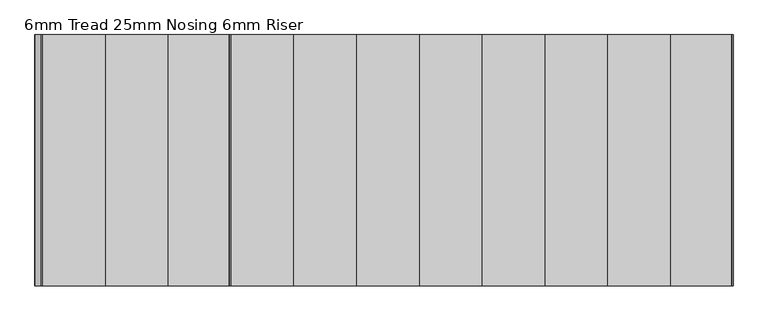
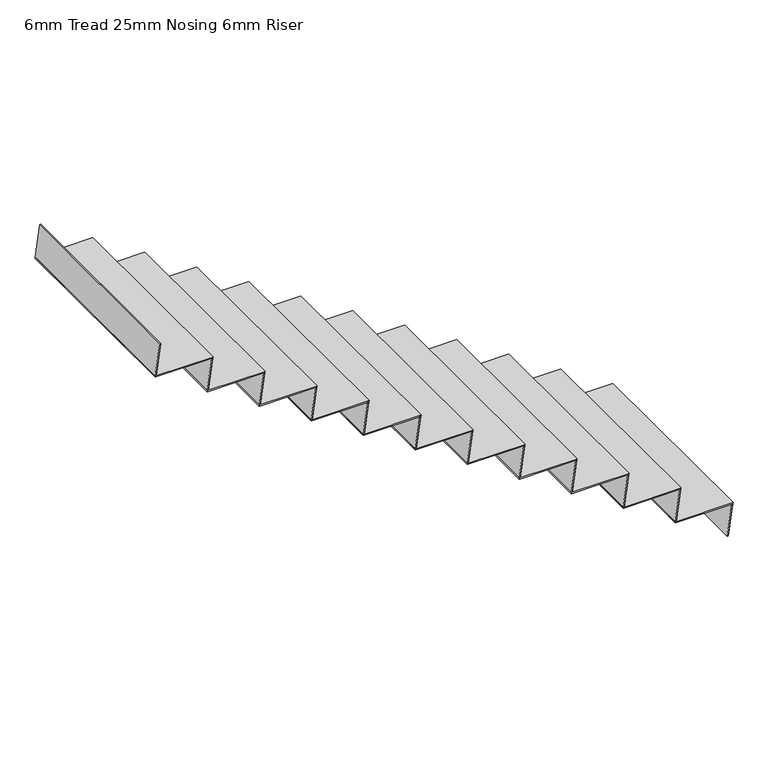
"""IFC4 building model written with IfcOpenShell, lengths in millimetres: stair flight geometry, 6mm Tread 25mm Nosing 6mm Riser."""

from ifc_helpers import new_model, si_unit, frame, origin, place, context, project, spatial, polyline, outline, extrude, source, transform, mapped, element, save


def stair_flight_6mm_tread_25mm_nosing_6mm_riser_325804f1(model_context):
    return source(origin(), model_context, "Body", "SweptSolid", [
        extrude(outline(polyline([(2133.3333333, 16350.0), (2133.3333333, 16043.9409643), (2127.3333333, 16043.0972143), (2127.3333333, 16349.15625), (2133.3333333, 16350.0)])), frame((0.0, 12030.4345331, 0.0), z_axis=(0.0, 1.0, 0.0), x_axis=(0.0, 0.0, 1.0)), (0.0, 0.0, 1.0), 1100.0),
        extrude(outline(polyline([(2127.3333333, 16349.15625), (2127.3333333, 16343.0972143), (1955.5555556, 16318.9409643), (1955.5555556, 16325.0), (2127.3333333, 16349.15625)])), frame((0.0, 12030.4345331, 0.0), z_axis=(0.0, 1.0, 0.0), x_axis=(0.0, 0.0, 1.0)), (0.0, 0.0, 1.0), 1100.0),
        extrude(outline(polyline([(2305.1111111, 16074.15625), (2305.1111111, 16068.0972143), (2133.3333333, 16043.9409643), (2133.3333333, 16050.0), (2305.1111111, 16074.15625)])), frame((0.0, 12030.4345331, 0.0), z_axis=(0.0, 1.0, 0.0), x_axis=(0.0, 0.0, 1.0)), (0.0, 0.0, 1.0), 1100.0),
        extrude(outline(polyline([(2311.1111111, 16075.0), (2311.1111111, 15768.9409643), (2305.1111111, 15768.0972143), (2305.1111111, 16074.15625), (2311.1111111, 16075.0)])), frame((0.0, 12030.4345331, 0.0), z_axis=(0.0, 1.0, 0.0), x_axis=(0.0, 0.0, 1.0)), (0.0, 0.0, 1.0), 1100.0),
        extrude(outline(polyline([(2482.8888889, 15799.15625), (2482.8888889, 15793.0972143), (2311.1111111, 15768.9409643), (2311.1111111, 15775.0), (2482.8888889, 15799.15625)])), frame((0.0, 12030.4345331, 0.0), z_axis=(0.0, 1.0, 0.0), x_axis=(0.0, 0.0, 1.0)), (0.0, 0.0, 1.0), 1100.0),
        extrude(outline(polyline([(2488.8888889, 15800.0), (2488.8888889, 15493.9409643), (2482.8888889, 15493.0972143), (2482.8888889, 15799.15625), (2488.8888889, 15800.0)])), frame((0.0, 12030.4345331, 0.0), z_axis=(0.0, 1.0, 0.0), x_axis=(0.0, 0.0, 1.0)), (0.0, 0.0, 1.0), 1100.0),
        extrude(outline(polyline([(2660.6666667, 15524.15625), (2660.6666667, 15518.0972143), (2488.8888889, 15493.9409643), (2488.8888889, 15500.0), (2660.6666667, 15524.15625)])), frame((0.0, 12030.4345331, 0.0), z_axis=(0.0, 1.0, 0.0), x_axis=(0.0, 0.0, 1.0)), (0.0, 0.0, 1.0), 1100.0),
        extrude(outline(polyline([(2666.6666667, 15525.0), (2666.6666667, 15218.9409643), (2660.6666667, 15218.0972143), (2660.6666667, 15524.15625), (2666.6666667, 15525.0)])), frame((0.0, 12030.4345331, 0.0), z_axis=(0.0, 1.0, 0.0), x_axis=(0.0, 0.0, 1.0)), (0.0, 0.0, 1.0), 1100.0),
        extrude(outline(polyline([(2838.4444444, 15249.15625), (2838.4444444, 15243.0972143), (2666.6666667, 15218.9409643), (2666.6666667, 15225.0), (2838.4444444, 15249.15625)])), frame((0.0, 12030.4345331, 0.0), z_axis=(0.0, 1.0, 0.0), x_axis=(0.0, 0.0, 1.0)), (0.0, 0.0, 1.0), 1100.0),
        extrude(outline(polyline([(2844.4444444, 15250.0), (2844.4444444, 14943.9409643), (2838.4444444, 14943.0972143), (2838.4444444, 15249.15625), (2844.4444444, 15250.0)])), frame((0.0, 12030.4345331, 0.0), z_axis=(0.0, 1.0, 0.0), x_axis=(0.0, 0.0, 1.0)), (0.0, 0.0, 1.0), 1100.0),
        extrude(outline(polyline([(3016.2222222, 14974.15625), (3016.2222222, 14968.0972143), (2844.4444444, 14943.9409643), (2844.4444444, 14950.0), (3016.2222222, 14974.15625)])), frame((0.0, 12030.4345331, 0.0), z_axis=(0.0, 1.0, 0.0), x_axis=(0.0, 0.0, 1.0)), (0.0, 0.0, 1.0), 1100.0),
        extrude(outline(polyline([(3022.2222222, 14975.0), (3022.2222222, 14668.9409643), (3016.2222222, 14668.0972143), (3016.2222222, 14974.15625), (3022.2222222, 14975.0)])), frame((0.0, 12030.4345331, 0.0), z_axis=(0.0, 1.0, 0.0), x_axis=(0.0, 0.0, 1.0)), (0.0, 0.0, 1.0), 1100.0),
        extrude(outline(polyline([(3194.0, 14699.15625), (3194.0, 14693.0972143), (3022.2222222, 14668.9409643), (3022.2222222, 14675.0), (3194.0, 14699.15625)])), frame((0.0, 12030.4345331, 0.0), z_axis=(0.0, 1.0, 0.0), x_axis=(0.0, 0.0, 1.0)), (0.0, 0.0, 1.0), 1100.0),
        extrude(outline(polyline([(3200.0, 14700.0), (3200.0, 14393.9409643), (3194.0, 14393.0972143), (3194.0, 14699.15625), (3200.0, 14700.0)])), frame((0.0, 12030.4345331, 0.0), z_axis=(0.0, 1.0, 0.0), x_axis=(0.0, 0.0, 1.0)), (0.0, 0.0, 1.0), 1100.0),
        extrude(outline(polyline([(3371.7777778, 14424.15625), (3371.7777778, 14418.0972143), (3200.0, 14393.9409643), (3200.0, 14400.0), (3371.7777778, 14424.15625)])), frame((0.0, 12030.4345331, 0.0), z_axis=(0.0, 1.0, 0.0), x_axis=(0.0, 0.0, 1.0)), (0.0, 0.0, 1.0), 1100.0),
        extrude(outline(polyline([(3377.7777778, 14425.0), (3377.7777778, 14118.9409643), (3371.7777778, 14118.0972143), (3371.7777778, 14424.15625), (3377.7777778, 14425.0)])), frame((0.0, 12030.4345331, 0.0), z_axis=(0.0, 1.0, 0.0), x_axis=(0.0, 0.0, 1.0)), (0.0, 0.0, 1.0), 1100.0),
        extrude(outline(polyline([(3549.5555556, 14149.15625), (3549.5555556, 14143.0972143), (3377.7777778, 14118.9409643), (3377.7777778, 14125.0), (3549.5555556, 14149.15625)])), frame((0.0, 12030.4345331, 0.0), z_axis=(0.0, 1.0, 0.0), x_axis=(0.0, 0.0, 1.0)), (0.0, 0.0, 1.0), 1100.0),
        extrude(outline(polyline([(3555.5555556, 14150.0), (3555.5555556, 13843.9409643), (3549.5555556, 13843.0972143), (3549.5555556, 14149.15625), (3555.5555556, 14150.0)])), frame((0.0, 12030.4345331, 0.0), z_axis=(0.0, 1.0, 0.0), x_axis=(0.0, 0.0, 1.0)), (0.0, 0.0, 1.0), 1100.0),
        extrude(outline(polyline([(3727.3333333, 13874.15625), (3727.3333333, 13868.0972143), (3555.5555556, 13843.9409643), (3555.5555556, 13850.0), (3727.3333333, 13874.15625)])), frame((0.0, 12030.4345331, 0.0), z_axis=(0.0, 1.0, 0.0), x_axis=(0.0, 0.0, 1.0)), (0.0, 0.0, 1.0), 1100.0),
        extrude(outline(polyline([(3733.3333333, 13875.0), (3733.3333333, 13568.9409643), (3727.3333333, 13568.0972143), (3727.3333333, 13874.15625), (3733.3333333, 13875.0)])), frame((0.0, 12030.4345331, 0.0), z_axis=(0.0, 1.0, 0.0), x_axis=(0.0, 0.0, 1.0)), (0.0, 0.0, 1.0), 1100.0),
        extrude(outline(polyline([(3905.1111111, 13599.15625), (3905.1111111, 13593.0972143), (3733.3333333, 13568.9409643), (3733.3333333, 13575.0), (3905.1111111, 13599.15625)])), frame((0.0, 12030.4345331, 0.0), z_axis=(0.0, 1.0, 0.0), x_axis=(0.0, 0.0, 1.0)), (0.0, 0.0, 1.0), 1100.0),
        extrude(outline(polyline([(4082.8888889, 13324.15625), (4082.8888889, 13318.0972143), (3911.1111111, 13293.9409643), (3911.1111111, 13300.0), (4082.8888889, 13324.15625)])), frame((0.0, 12030.4345331, 0.0), z_axis=(0.0, 1.0, 0.0), x_axis=(0.0, 0.0, 1.0)), (0.0, 0.0, 1.0), 1100.0),
        extrude(outline(polyline([(3911.1111111, 13600.0), (3911.1111111, 13293.9409643), (3905.1111111, 13293.0972143), (3905.1111111, 13599.15625), (3911.1111111, 13600.0)])), frame((0.0, 12030.4345331, 0.0), z_axis=(0.0, 1.0, 0.0), x_axis=(0.0, 0.0, 1.0)), (0.0, 0.0, 1.0), 1100.0),
    ])


if __name__ == "__main__":
    model = new_model("IFC4")
    model_context = context("Model", 3, world=origin())
    ifc_project = project(units=[si_unit("LENGTHUNIT", "METRE", prefix="MILLI")], contexts=[model_context])
    site = spatial("IfcSite", under=ifc_project)
    building = spatial("IfcBuilding", under=site)
    placement = place(None, origin())
    stair_flight_6mm_tread_25mm_nosing_6mm_riser_shape = stair_flight_6mm_tread_25mm_nosing_6mm_riser_325804f1(model_context)
    element("IfcStairFlight", 1, ObjectType="6mm Tread 25mm Nosing 6mm Riser", at=placement, inside=building, context=model_context, shape_type="MappedRepresentation", body=[
        mapped(stair_flight_6mm_tread_25mm_nosing_6mm_riser_shape, transform((0.0, 0.0, 0.0), x_axis=(1.0, 0.0, 0.0), y_axis=(0.0, 1.0, 0.0), z_axis=(0.0, 0.0, 1.0))),
    ])
    save(model, "model.ifc")

# Revit data of these elements
# Element 1 (IfcStairFlight, "6mm Tread 25mm Nosing 6mm Riser")
#   Materials on its faces: "Steel, Paint Finish, Dark Gray"
# Materials
#   "Steel, Paint Finish, Dark Gray": class "Metal", colour RGB 89 89 89, transparency 0, Description = "Steel, paint finish, dark gray, glossy", Cost = 0
